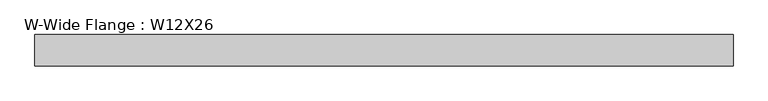
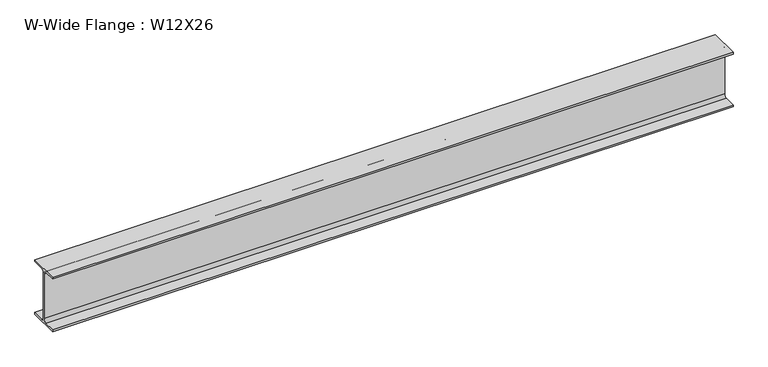
"""IFC4 building model written with IfcOpenShell, lengths in millimetres: beam geometry, W-Wide Flange : W12X26."""

from ifc_helpers import new_model, si_unit, point, frame, frame_2d, origin, place, context, project, spatial, polyline, circle_curve, trimmed, segment, composite_curve, outline, extrude, source, transform, mapped, element, save


def w_wide_flange_w12x26_2398d520(model_context):
    return source(origin(), model_context, "Body", "SweptSolid", [
        extrude(outline(composite_curve([segment(polyline([(82.423, -145.288), (82.423, -154.94), (-82.423, -154.94), (-82.423, -145.288), (-20.2565, -145.288)]), True, "CONTINUOUS"), segment(trimmed(circle_curve(frame_2d((-20.2565, -127.9525)), 17.3355), [point((-20.2565, -145.288))], [point((-2.921, -127.9525))], True, "CARTESIAN"), True, "CONTINUOUS"), segment(polyline([(-2.921, -127.9525), (-2.921, 127.9525)]), True, "CONTINUOUS"), segment(trimmed(circle_curve(frame_2d((-20.2565, 127.9525)), 17.3355), [point((-2.921, 127.9525))], [point((-20.2565, 145.288))], True, "CARTESIAN"), True, "CONTINUOUS"), segment(polyline([(-20.2565, 145.288), (-82.423, 145.288), (-82.423, 154.94), (82.423, 154.94), (82.423, 145.288), (20.2565, 145.288)]), True, "CONTINUOUS"), segment(trimmed(circle_curve(frame_2d((20.2565, 127.9525)), 17.3355), [point((20.2565, 145.288))], [point((2.921, 127.9525))], True, "CARTESIAN"), True, "CONTINUOUS"), segment(polyline([(2.921, 127.9525), (2.921, -127.9525)]), True, "CONTINUOUS"), segment(trimmed(circle_curve(frame_2d((20.2565, -127.9525)), 17.3355), [point((2.921, -127.9525))], [point((20.2565, -145.288))], True, "CARTESIAN"), True, "CONTINUOUS"), segment(polyline([(20.2565, -145.288), (82.423, -145.288)]), True, "CONTINUOUS")], self_intersect=False)), frame((-1774.8760943, 0.0, 0.0), z_axis=(1.0, 0.0, 0.0), x_axis=(0.0, 1.0, 0.0)), (0.0, 0.0, 1.0), 3670.3),
    ])


if __name__ == "__main__":
    model = new_model("IFC4")
    model_context = context("Model", 3, world=origin())
    ifc_project = project(units=[si_unit("LENGTHUNIT", "METRE", prefix="MILLI")], contexts=[model_context])
    site = spatial("IfcSite", under=ifc_project)
    building = spatial("IfcBuilding", under=site)
    placement = place(None, origin())
    w_wide_flange_w12x26_shape = w_wide_flange_w12x26_2398d520(model_context)
    element("IfcBeam", 1, ObjectType="W-Wide Flange : W12X26", at=placement, inside=building, context=model_context, shape_type="MappedRepresentation", body=[
        mapped(w_wide_flange_w12x26_shape, transform((0.0, 0.0, 0.0), x_axis=(1.0, 0.0, 0.0), y_axis=(0.0, 1.0, 0.0), z_axis=(0.0, 0.0, 1.0))),
    ])
    save(model, "model.ifc")

# Revit data of these elements
# Type "W-Wide Flange : W12X26"
#   Assembly Code = "B10"
#   W = 26
#   Length [instance default] = 5' - 0"
#   bf = 0' - 6.49"
#   d = 1' - 0.2"
#   k = 0' - 1 1/16"
#   k2 = 0' - 0.6825"
#   tf = 0' - 0.38"
#   tw = 0' - 0.23"
#   A = 0.053125 SF
#   Structural Material [instance default] = Steel ASTM A992
# Element 1 (IfcBeam, "W-Wide Flange : W12X26")
#   Materials on its faces: "Steel ASTM A992"
# Materials
#   "Steel ASTM A992": class "Metal", colour RGB 199 199 199, transparency 0, Description = "Structural steel 50ksi", Cost = 0
